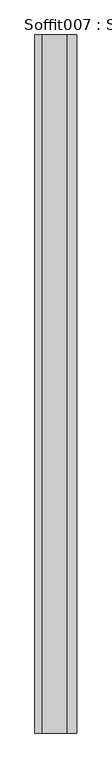
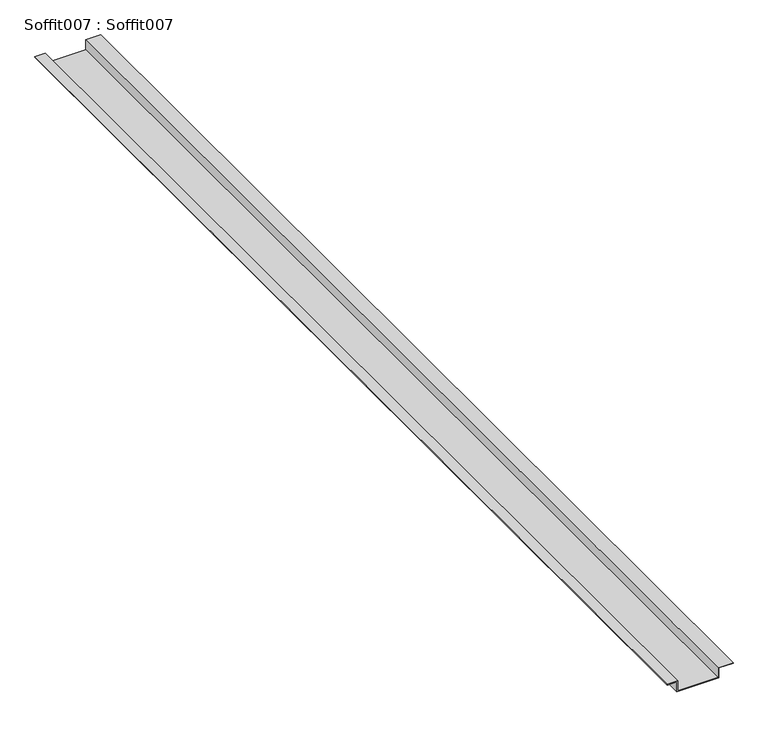
"""IFC4 building model written with IfcOpenShell, lengths in millimetres: proxy geometry, Soffit007 : Soffit007."""

from ifc_helpers import new_model, si_unit, frame, origin, place, context, project, spatial, polyline, outline, extrude, source, transform, mapped, element, save


def soffit007_soffit007_9be96442(model_context):
    return source(origin(), model_context, "Body", "SweptSolid", [
        extrude(outline(polyline([(39560.2460083, -9735.5897631), (39558.9760083, -9735.5897631), (39558.9760083, -9717.7304687), (39539.8868001, -9717.7304687), (39539.8868001, -9641.5317206), (39558.976008, -9641.5317206), (39558.976008, -9615.2760935), (39560.246008, -9615.2760935), (39560.246008, -9642.8017206), (39541.1567168, -9642.8017206), (39541.1567168, -9716.4603855), (39560.2460083, -9716.4603855), (39560.2460083, -9735.5897631)])), frame((0.0, 7982.1531721, 0.0), z_axis=(0.0, 1.0, 0.0), x_axis=(0.0, 0.0, 1.0)), (0.0, 0.0, 1.0), 2000.0),
    ])


if __name__ == "__main__":
    model = new_model("IFC4")
    model_context = context("Model", 3, world=origin())
    ifc_project = project(units=[si_unit("LENGTHUNIT", "METRE", prefix="MILLI")], contexts=[model_context])
    site = spatial("IfcSite", under=ifc_project)
    building = spatial("IfcBuilding", under=site)
    placement = place(None, origin())
    soffit007_soffit007_shape = soffit007_soffit007_9be96442(model_context)
    element("IfcBuildingElementProxy", 1, Name="Soffit007 : Soffit007", ObjectType="Soffit007 : Soffit007", at=placement, inside=building, context=model_context, shape_type="MappedRepresentation", body=[
        mapped(soffit007_soffit007_shape, transform((0.0, 0.0, 0.0), x_axis=(1.0, 0.0, 0.0), y_axis=(0.0, 1.0, 0.0), z_axis=(0.0, 0.0, 1.0))),
    ])
    save(model, "model.ifc")

# Revit data of these elements
# Type "Soffit007 : Soffit007"
#   NameOverride = "Soffit007"
# Element 1 (IfcBuildingElementProxy, "Soffit007 : Soffit007")
#   Materials on its faces: "16 GA. COPPER SOFFIT VENT - VERIFY W/ ARCHITECT ON LOCATION"
# Materials
#   "16 GA. COPPER SOFFIT VENT - VERIFY W/ ARCHITECT ON LOCATION": class "Unassigned", colour RGB 85 255 127, transparency 0
